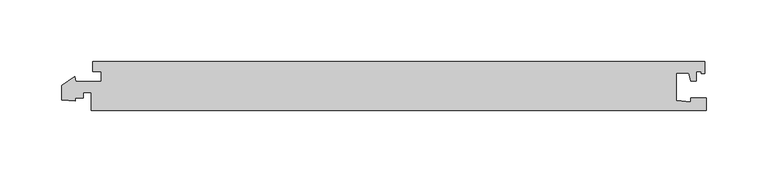
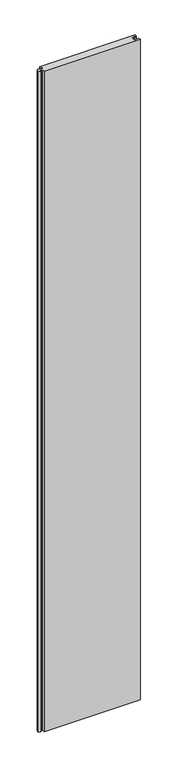
"""IFC4 building model written with IfcOpenShell, lengths in millimetres: proxy geometry, Generic Models 5:Generic Models 5:321804:Generic Models 5:321804 : Generic Models 5:Generic Models 5:321804:4 : Generic Models 5:Generic Models 5:321804:Generic Models 5:321804 : Generic Models 5:Generic Models 5:321804:300761."""

from ifc_helpers import new_model, si_unit, frame, origin, place, context, project, spatial, polyline, outline, extrude, source, transform, mapped, element, save


def generic_models_40f12c52(model_context):
    return source(origin(), model_context, "Body", "SweptSolid", [
        extrude(outline(polyline([(593294.8386129, -568238.0537319), (593284.4802827, -568238.0537319), (593284.4802827, -568260.5495221), (593296.4802827, -568261.5993861), (593296.4802827, -568258.3537319), (593309.2302827, -568258.3537319), (593309.2302827, -568268.5537319), (592809.2302827, -568268.5537319), (592809.2302827, -568254.0537319), (592802.6052827, -568254.0537319), (592802.6052827, -568258.3537319), (592795.9802827, -568258.3537319), (592795.9802827, -568261.0537319), (592784.9802827, -568260.0913566), (592784.9802827, -568248.2332156), (592795.6617846, -568241.1258504), (592796.7142572, -568245.0537319), (592817.4302827, -568245.0537319), (592817.4302827, -568237.0537319), (592810.4802827, -568237.0537319), (592810.4802827, -568228.5537319), (593307.9802827, -568228.5537319), (593307.9802827, -568238.5537319), (593304.9802827, -568238.5537319), (593304.9802827, -568237.0537319), (593301.0302827, -568237.0537319), (593301.0302827, -568244.5537319), (593296.5802827, -568244.5537319), (593294.8386129, -568238.0537319)])), frame((0.0, 0.0, 4883.8301003), z_axis=(0.0, 0.0, 1.0), x_axis=(1.0, 0.0, 0.0)), (0.0, 0.0, 1.0), 3634.8310765),
    ])


if __name__ == "__main__":
    model = new_model("IFC4")
    model_context = context("Model", 3, world=origin())
    ifc_project = project(units=[si_unit("LENGTHUNIT", "METRE", prefix="MILLI")], contexts=[model_context])
    site = spatial("IfcSite", under=ifc_project)
    building = spatial("IfcBuilding", under=site)
    placement = place(None, origin())
    generic_models_shape = generic_models_40f12c52(model_context)
    element("IfcBuildingElementProxy", 1, Name="Generic Models 5:Generic Models 5:321804:Generic Models 5:321804 : Generic Models 5:Generic Models 5:321804:4 : Generic Models 5:Generic Models 5:321804:Generic Models 5:321804 : Generic Models 5:Generic Models 5:321804:300761", ObjectType="Generic Models 5:Generic Models 5:321804:Generic Models 5:321804 : Generic Models 5:Generic Models 5:321804:4 : Generic Models 5:Generic Models 5:321804:Generic Models 5:321804 : Generic Models 5:Generic Models 5:321804:300761", at=placement, inside=building, context=model_context, shape_type="MappedRepresentation", body=[
        mapped(generic_models_shape, transform((0.0, 0.0, 0.0), x_axis=(1.0, 0.0, 0.0), y_axis=(0.0, 1.0, 0.0), z_axis=(0.0, 0.0, 1.0))),
    ])
    save(model, "model.ifc")

# Revit data of these elements
# Type "Generic Models 5:Generic Models 5:321804:Generic Models 5:321804 : Generic Models 5:Generic Models 5:321804:4 : Generic Models 5:Generic Models 5:321804:Generic Models 5:321804 : Generic Models 5:Generic Models 5:321804:300761"
#   NameOverride = "Generic Models 5:Generic Models 5:321804:Generic Models 5:321804 : Generic Models 5:Generic Models 5:321804:300761"
#   ObjectTypeOverride = "Generic Models 5:321804 : Generic Models 5:Generic Models 5:321804"
#   Reference = "Generic Models 5"
#   Tag = "300761"
# Element 1 (IfcBuildingElementProxy, "Generic Models 5:Generic Models 5:321804:Generic Models 5:321804 : Generic Models 5:Generic Models 5:321804:4 : Generic Models 5:Generic Models 5:321804:Generic Models 5:321804 : Generic Models 5:Generic Models 5:321804:300761")
#   Materials on its faces: "POLYCARBONATE PANEL - ARCOPLUS 547"
# Materials
#   "POLYCARBONATE PANEL - ARCOPLUS 547": class "Unassigned", colour RGB 202 225 249, transparency 0.45, Cost = 0
